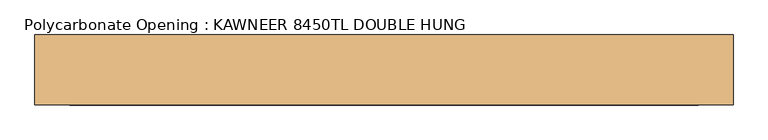
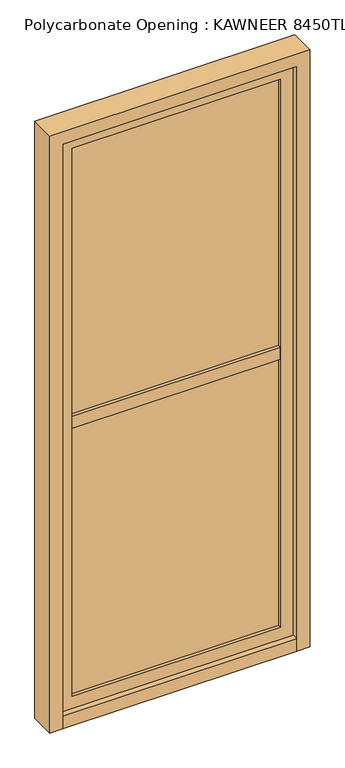
"""IFC4 building model written with IfcOpenShell, lengths in millimetres: door geometry, Polycarbonate Opening : KAWNEER 8450TL DOUBLE HUNG."""

from ifc_helpers import new_model, si_unit, frame, origin, origin_with_axes, place, context, project, spatial, polyline, outline, extrude, source, transform, mapped, element, save


def polycarbonate_opening_kawneer_8450tl_double_hung_191c6181(model_context):
    return source(origin(), model_context, "Body", "SweptSolid", [
        extrude(outline(polyline([(457.2, -12.7), (-457.2, -12.7), (-457.2, 12.7), (457.2, 12.7), (457.2, -12.7)])), frame((0.0, 0.0, 50.8), z_axis=(0.0, 0.0, 1.0), x_axis=(1.0, 0.0, 0.0)), (0.0, 0.0, 1.0), 2360.0132885),
        extrude(outline(polyline([(2410.8132885, -457.2), (0.0, -457.2), (0.0, 457.2), (2410.8132885, 457.2), (2410.8132885, -457.2)]), holes=[polyline([(101.6, 406.4), (101.6, -406.4), (2360.0132885, -406.4), (2360.0132885, 406.4), (101.6, 406.4)])]), frame((0.0, -25.4, 0.0), z_axis=(0.0, 1.0, 0.0), x_axis=(0.0, 0.0, 1.0)), (0.0, 0.0, 1.0), 50.8),
        extrude(outline(polyline([(2461.6132885, 508.0), (2461.6132885, -508.0), (0.0, -508.0), (0.0, -457.2), (2410.8132885, -457.2), (2410.8132885, 457.2), (0.0, 457.2), (0.0, 508.0), (2461.6132885, 508.0)])), frame((0.0, -50.8, 0.0), z_axis=(0.0, 1.0, 0.0), x_axis=(0.0, 0.0, 1.0)), (0.0, 0.0, 1.0), 101.6),
        extrude(outline(polyline([(457.2, -50.8), (-457.2, -50.8), (-457.2, 50.8), (457.2, 50.8), (457.2, -50.8)])), origin_with_axes(), (0.0, 0.0, 1.0), 50.8),
        extrude(outline(polyline([(406.4, -25.4), (-406.4, -25.4), (-406.4, 25.4), (406.4, 25.4), (406.4, -25.4)])), frame((0.0, 0.0, 1205.4066443), z_axis=(0.0, 0.0, 1.0), x_axis=(1.0, 0.0, 0.0)), (0.0, 0.0, 1.0), 50.8),
    ])


if __name__ == "__main__":
    model = new_model("IFC4")
    model_context = context("Model", 3, world=origin())
    ifc_project = project(units=[si_unit("LENGTHUNIT", "METRE", prefix="MILLI")], contexts=[model_context])
    site = spatial("IfcSite", under=ifc_project)
    building = spatial("IfcBuilding", under=site)
    placement = place(None, origin())
    polycarbonate_opening_kawneer_8450tl_double_hung_shape = polycarbonate_opening_kawneer_8450tl_double_hung_191c6181(model_context)
    element("IfcDoor", 1, ObjectType="Polycarbonate Opening : KAWNEER 8450TL DOUBLE HUNG", at=placement, inside=building, context=model_context, shape_type="MappedRepresentation", body=[
        mapped(polycarbonate_opening_kawneer_8450tl_double_hung_shape, transform((0.0, 0.0, 0.0), x_axis=(1.0, 0.0, 0.0), y_axis=(0.0, 1.0, 0.0), z_axis=(0.0, 0.0, 1.0))),
    ])
    save(model, "model.ifc")

# Revit data of these elements
# Type "Polycarbonate Opening : KAWNEER 8450TL DOUBLE HUNG"
#   Type Mark = "59"
#   OD_DS_Door_Material = "ALUM./GLAZING"
#   OD_DS_Door_Type = "STOREFRONT - DOUBLE HUNG WINDOW"
#   OD_DS_Lockset = "POLE OPERATOR HARDWARE FOR TOP SASH; BOTTOM SASH MECHANICALLY FIXED"
#   Analytic Construction = "<None>"
#   offset [instance default] = 0' - 2"
#   Stile = 0' - 2"
#   Mullion Width = 0' - 2"
#   Mullion Depth = 0' - 4"
#   Opening Size [instance default] = 5' - 1.50212"
#   Door Width [instance default] = 5' - 1.50212"
#   Window ON/OFF = no
#   Door On/Off = yes
#   Mullion Material = DOUBLE HUNG (CLEAR ANODIZED ALUM) - TEMPERED INSULATED GLAZING (CARDINAL GLASS LoĒ²-240\nOR EQUIVALENT)
#   Glass Material = TEMPERED INSULATED GLAZING (CARDINAL GLASS LoĒ²-240\nOR EQUIVALENT)
#   Door Material = DOUBLE HUNG (CLEAR ANODIZED ALUM) - TEMPERED INSULATED GLAZING (CARDINAL GLASS LoĒ²-240\nOR EQUIVALENT)
# Element 1 (IfcDoor, "Polycarbonate Opening : KAWNEER 8450TL DOUBLE HUNG")
#   offset = 0' - 0"
#   Materials on its faces: "DOUBLE HUNG (CLEAR ANODIZED ALUM) - TEMPERED INSULATED GLAZING (CARDINAL GLASS LoĒ²-240\nOR EQUIVALENT)", "TEMPERED INSULATED GLAZING (CARDINAL GLASS LoĒ²-240\nOR EQUIVALENT)"
# Materials
#   "DOUBLE HUNG (CLEAR ANODIZED ALUM) - TEMPERED INSULATED GLAZING (CARDINAL GLASS LoĒ²-240\nOR EQUIVALENT)": class "Metal", colour RGB 244 244 244, transparency 0, Description = "Aluminum 6061", Cost = 0
#   "TEMPERED INSULATED GLAZING (CARDINAL GLASS LoĒ²-240\nOR EQUIVALENT)": class "Glass", colour RGB 196 205 210, transparency 0.85, Description = "Soda Lime Glass", Cost = 0
